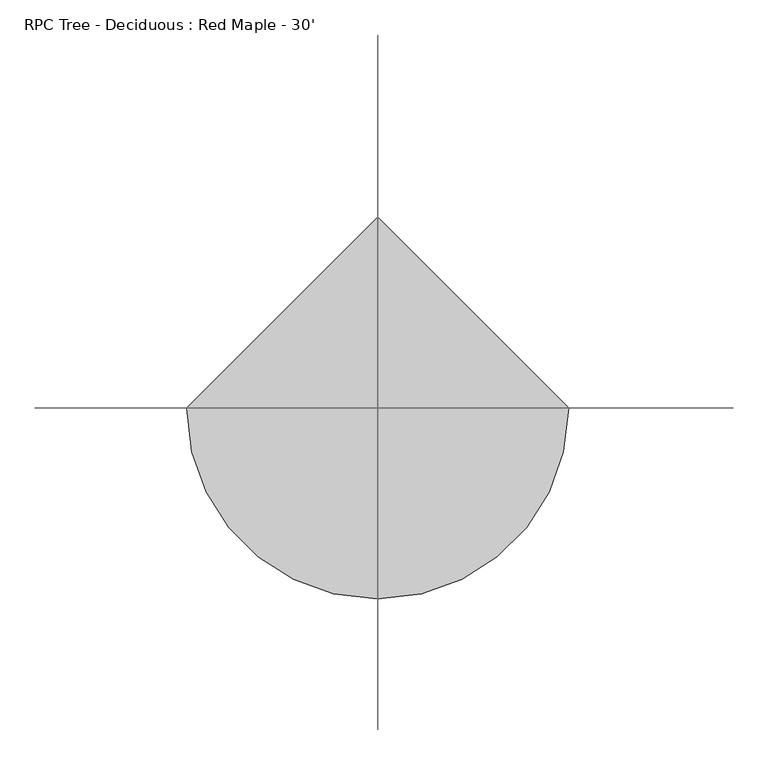
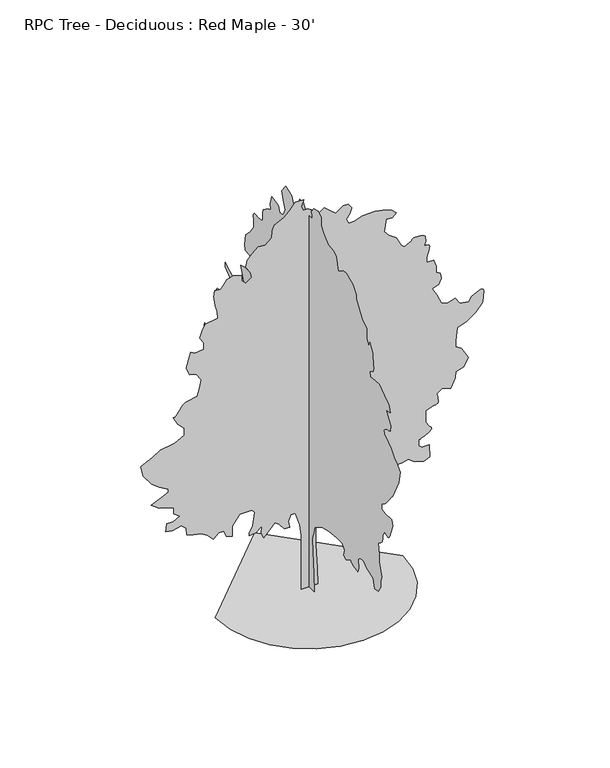
"""IFC4 building model written with IfcOpenShell, lengths in millimetres: geographic element geometry, RPC Tree - Deciduous : Red Maple - 30'."""

import ifcopenshell
import ifcopenshell.guid

model = None  # the IFC model being written
_history = None  # IfcOwnerHistory: only IFC2X3 demands one
_inside = {}  # id of a spatial element -> (the spatial element, [elements in it])
_under = {}  # id of a project, library or spatial element -> (it, [spatial elements below it])
_declared = {}  # id of a project -> (the project, [libraries it declares])
_typed = {}  # id of a type object -> (the type object, [elements of that type])
_made_of = {}  # id of a material, layer set ... -> (it, [elements and type objects made of it])


def new_model(schema):
    """Start an empty IFC model of exactly this schema.

    Asked for "IFC4X3", IfcOpenShell would pick the latest addendum, in which some entities
    have other attributes; the version numbers below select the first issue.
    IFC2X3 requires an IfcOwnerHistory on every rooted entity: one is made here for all.
    """
    global model, _history
    if schema == "IFC4X3":
        model = ifcopenshell.file(schema_version=(4, 3, 0, 0))
    else:
        model = ifcopenshell.file(schema=schema)
    _inside.clear()
    _under.clear()
    _declared.clear()
    _typed.clear()
    _made_of.clear()
    _history = None
    if model.schema == "IFC2X3":
        org = make("IfcOrganization", Name="unknown")
        user = make(
            "IfcPersonAndOrganization",
            ThePerson=make("IfcPerson", FamilyName="unknown"),
            TheOrganization=org,
        )
        app = make(
            "IfcApplication",
            ApplicationDeveloper=org,
            Version="unknown",
            ApplicationFullName="unknown",
            ApplicationIdentifier="unknown",
        )
        _history = make(
            "IfcOwnerHistory",
            OwningUser=user,
            OwningApplication=app,
            ChangeAction="ADDED",
            CreationDate=0,
        )
    return model


def make(cls, **values):
    """One entity of the class cls with the attributes given. An attribute that is None is left unset."""
    return model.create_entity(
        cls, **{name: value for name, value in values.items() if value is not None}
    )


def rooted(cls, **values):
    """An entity with a GlobalId (a new one), such as an element, a storey or a relation."""
    return make(cls, GlobalId=ifcopenshell.guid.new(), OwnerHistory=_history, **values)


def si_unit(unit_type, name, prefix=None):
    """IfcSIUnit, for example si_unit("LENGTHUNIT", "METRE", prefix="MILLI")."""
    return make("IfcSIUnit", UnitType=unit_type, Prefix=prefix, Name=name)


def assignment(units):
    """IfcUnitAssignment: the units of a project."""
    return None if units is None else make("IfcUnitAssignment", Units=units)


def point(xyz):
    """IfcCartesianPoint."""
    return None if xyz is None else make("IfcCartesianPoint", Coordinates=xyz)


def direction(xyz):
    """IfcDirection."""
    return None if xyz is None else make("IfcDirection", DirectionRatios=xyz)


def frame(location, z_axis=None, x_axis=None):
    """IfcAxis2Placement3D, a coordinate frame: its origin and axes. An axis left out is left unset."""
    return make(
        "IfcAxis2Placement3D",
        Location=point(location),
        Axis=direction(z_axis),
        RefDirection=direction(x_axis),
    )


def origin():
    """The frame at (0, 0, 0) with its axes left unset."""
    return frame((0.0, 0.0, 0.0))


def place(relative_to, where):
    """IfcLocalPlacement: puts the frame where relative to a parent placement (None: the world)."""
    return make(
        "IfcLocalPlacement", PlacementRelTo=relative_to, RelativePlacement=where
    )


def context(
    kind, dimensions, precision=None, world=None, true_north=None, identifier=None
):
    """IfcGeometricRepresentationContext, for example the 3D "Model" context."""
    return make(
        "IfcGeometricRepresentationContext",
        ContextIdentifier=identifier,
        ContextType=kind,
        CoordinateSpaceDimension=dimensions,
        Precision=precision,
        WorldCoordinateSystem=world,
        TrueNorth=true_north,
    )


def project(units=None, contexts=None):
    """IfcProject with its units and contexts."""
    return rooted(
        "IfcProject",
        Name="project",
        RepresentationContexts=contexts,
        UnitsInContext=assignment(units),
    )


def spatial(cls, under=None, at=None, **own):
    """A site, building, storey or space (cls), placed at a placement, below another one or the project."""
    s = rooted(cls, ObjectPlacement=at, **own)
    if under is not None:
        _under.setdefault(under.id(), (under, []))[1].append(s)
    return s


def point_list(points):
    """IfcCartesianPointList2D or 3D."""
    cls = (
        "IfcCartesianPointList2D" if len(points[0]) == 2 else "IfcCartesianPointList3D"
    )
    return make(cls, CoordList=points)


def triangles(points, corners, closed=None, point_numbers=None):
    """IfcTriangulatedFaceSet: each triangle names its three corners, points numbered from 1."""
    return make(
        "IfcTriangulatedFaceSet",
        Coordinates=point_list(points),
        Closed=closed,
        CoordIndex=corners,
        PnIndex=point_numbers,
    )


def shape(context_of_items, identifier, shape_type, items):
    """IfcShapeRepresentation: the items that make up one representation, for example the "Body"."""
    return make(
        "IfcShapeRepresentation",
        ContextOfItems=context_of_items,
        RepresentationIdentifier=identifier,
        RepresentationType=shape_type,
        Items=items,
    )


def source(mapping_origin, context_of_items, identifier, shape_type, items):
    """IfcRepresentationMap: a shape defined once, which mapped items show again and again."""
    return make(
        "IfcRepresentationMap",
        MappingOrigin=mapping_origin,
        MappedRepresentation=shape(context_of_items, identifier, shape_type, items),
    )


def transform(
    local_origin,
    x_axis=None,
    y_axis=None,
    z_axis=None,
    scale=None,
    scale2=None,
    scale3=None,
    uniform=True,
):
    """IfcCartesianTransformationOperator3D, or its non-uniform kind. x_axis, y_axis, z_axis: its Axis1, 2, 3."""
    if uniform:
        return make(
            "IfcCartesianTransformationOperator3D",
            Axis1=direction(x_axis),
            Axis2=direction(y_axis),
            LocalOrigin=point(local_origin),
            Scale=scale,
            Axis3=direction(z_axis),
        )
    return make(
        "IfcCartesianTransformationOperator3DnonUniform",
        Axis1=direction(x_axis),
        Axis2=direction(y_axis),
        LocalOrigin=point(local_origin),
        Scale=scale,
        Axis3=direction(z_axis),
        Scale2=scale2,
        Scale3=scale3,
    )


def mapped(mapping_source, mapping_target):
    """IfcMappedItem: shows the shape of a source again, moved by a transform."""
    return make(
        "IfcMappedItem", MappingSource=mapping_source, MappingTarget=mapping_target
    )


def made_of(thing, what):
    """Note that an element or type object is made of a material, layer set ...; save() writes the relation."""
    if what is not None:
        _made_of.setdefault(what.id(), (what, []))[1].append(thing)
    return thing


def element(
    cls,
    number,
    at=None,
    inside=None,
    cuts=None,
    type_object=None,
    material=None,
    context=None,
    identifier="Body",
    shape_type=None,
    held_by="IfcProductDefinitionShape",
    body=None,
    shapes=None,
    **own,
):
    """One element of the class cls, such as IfcWall. Its Tag is "e" and its number.

    at: its placement. inside: the storey or other place that contains it. cuts: it is an
    opening in that element (IfcRelVoidsElement). A single representation is given by context,
    identifier, shape_type and body (its items); several are given by shapes. held_by: the class
    of the entity that holds the representations. save() writes the other relations.
    """
    e = rooted(cls, Tag="e%d" % number, ObjectPlacement=at, **own)
    if body is not None:
        shapes = [shape(context, identifier, shape_type, body)]
    if shapes is not None:
        e.Representation = make(held_by, Representations=shapes)
    if inside is not None:
        _inside.setdefault(inside.id(), (inside, []))[1].append(e)
    if cuts is not None:
        rooted(
            "IfcRelVoidsElement", RelatingBuildingElement=cuts, RelatedOpeningElement=e
        )
    if type_object is not None:
        _typed.setdefault(type_object.id(), (type_object, []))[1].append(e)
    return made_of(e, material)


def aggregate(whole, parts):
    """IfcRelAggregates: a whole, such as a stair, and the parts it consists of."""
    return rooted("IfcRelAggregates", RelatingObject=whole, RelatedObjects=parts)


def save(model, path):
    """Write the relations noted so far, then the file.

    IfcRelAggregates (storeys below a building ...), IfcRelContainedInSpatialStructure (elements
    in a storey), IfcRelDefinesByType, IfcRelAssociatesMaterial and IfcRelDeclares: one each for
    every whole, place, type object, material and project.
    """
    for whole, parts in _under.values():
        aggregate(whole, parts)
    for where, things in _inside.values():
        rooted(
            "IfcRelContainedInSpatialStructure",
            RelatedElements=things,
            RelatingStructure=where,
        )
    for kind, things in _typed.values():
        rooted("IfcRelDefinesByType", RelatedObjects=things, RelatingType=kind)
    for what, things in _made_of.values():
        rooted("IfcRelAssociatesMaterial", RelatedObjects=things, RelatingMaterial=what)
    for by, libraries in _declared.values():
        rooted("IfcRelDeclares", RelatingContext=by, RelatedDefinitions=libraries)
    model.write(path)


def rpc_tree_deciduous_red_maple_30_cba750cc(model_context):
    return source(origin(), model_context, "Body", "Tessellation", [
        triangles([(5.9e-06, 200.5240248, 0.0131599), (5.9e-06, -200.5423013, 0.0131599), (5.9e-06, -173.8047255, 401.079007), (5.9e-06, -147.0663684, 922.4677488), (5.9e-06, -133.6980892, 1216.5822092), (5.9e-06, -173.8047255, 1363.6407475), (5.9e-06, -227.2806583, 1537.4352264), (5.9e-06, -320.8632274, 1590.9124855), (5.9e-06, -534.7644153, 1711.2323215), (5.9e-06, -762.0361897, 1764.7071098), (5.9e-06, -1069.5212002, 1804.8136734), (5.9e-06, -1283.4223881, 1804.8136734), (5.9e-06, -1377.0037399, 1697.8617714), (5.9e-06, -1336.897031, 1550.8033058), (5.9e-06, -1443.848933, 1510.6967422), (5.9e-06, -1617.6460281, 1604.2805649), (5.9e-06, -1620.762553, 1592.8200726), (5.9e-06, -1625.400642, 1581.362051), (5.9e-06, -1633.0790977, 1569.9041748), (5.9e-06, -1645.319339, 1558.4436825), (5.9e-06, -1663.6378429, 1546.9856609), (5.9e-06, -1689.5560284, 1535.5251686), (5.9e-06, -1724.595314, 1524.0672924), (5.9e-06, -1761.1942429, 1514.1662979), (5.9e-06, -1791.4812023, 1507.0721088), (5.9e-06, -1816.5027855, 1502.3197826), (5.9e-06, -1837.3156139, 1499.4343483), (5.9e-06, -1854.971077, 1497.9534794), (5.9e-06, -1870.5234707, 1497.4074371), (5.9e-06, -1885.021859, 1497.3286629), (5.9e-06, -1911.7604885, 1590.9124855), (5.9e-06, -1898.3924091, 1791.445594), (5.9e-06, -1978.6056816, 1871.6588665), (5.9e-06, -2112.293597, 1885.0269459), (5.9e-06, -2219.245499, 1778.0750439), (5.9e-06, -2473.2533958, 1697.8617714), (5.9e-06, -2540.1036758, 1497.3286629), (5.9e-06, -2660.4236572, 1510.6967422), (5.9e-06, -2767.3575371, 1671.125758), (5.9e-06, -2767.3575371, 1804.8136734), (5.9e-06, -2794.1038696, 1911.7655754), (5.9e-06, -2700.5302208, 2219.2479698), (5.9e-06, -2700.5302208, 2393.0450649), (5.9e-06, -2673.7838882, 2660.4236572), (5.9e-06, -2676.8572472, 2660.5759735), (5.9e-06, -2681.2261665, 2661.668058), (5.9e-06, -2688.1603363, 2664.6399696), (5.9e-06, -2698.9553169, 2670.4056061), (5.9e-06, -2714.9066689, 2679.9053169), (5.9e-06, -2737.284082, 2694.1038689), (5.9e-06, -2767.3575371, 2713.8904518), (5.9e-06, -2796.66912, 2738.3761665), (5.9e-06, -2816.8623642, 2765.6558968), (5.9e-06, -2829.4607231, 2795.2721123), (5.9e-06, -2835.9629425, 2826.7681549), (5.9e-06, -2837.9189278, 2859.6612053), (5.9e-06, -2836.8265526, 2893.4940239), (5.9e-06, -2834.2104332, 2927.8096619), (5.9e-06, -2914.423851, 3061.4898743), (5.9e-06, -2945.8434448, 3041.8556076), (5.9e-06, -2976.6790627, 3024.6598549), (5.9e-06, -3006.3211487, 3012.3917084), (5.9e-06, -3034.2357239, 3007.4641022), (5.9e-06, -3059.8135231, 3012.3917084), (5.9e-06, -3082.4449905, 3029.5618813), (5.9e-06, -3101.5964378, 3061.4898743), (5.9e-06, -3235.2766502, 3382.3429642), (5.9e-06, -3195.1700867, 3516.0231766), (5.9e-06, -2941.1698929, 3502.6629456), (5.9e-06, -2794.1038696, 3516.0231766), (5.9e-06, -2807.4641006, 3649.7289688), (5.9e-06, -2841.8811859, 3670.0236603), (5.9e-06, -2876.5523254, 3691.8420959), (5.9e-06, -2911.6551247, 3716.7088921), (5.9e-06, -2947.4692177, 3746.1475021), (5.9e-06, -2984.2230789, 3781.6566719), (5.9e-06, -3022.1707626, 3824.7604362), (5.9e-06, -3061.4898743, 3876.98283), (5.9e-06, -3098.0914192, 3928.4433517), (5.9e-06, -3128.3680595, 3969.3626564), (5.9e-06, -3153.3871719, 4001.5191238), (5.9e-06, -3174.2152611, 4026.6652634), (5.9e-06, -3191.8682533, 4046.5280045), (5.9e-06, -3207.412944, 4062.9110161), (5.9e-06, -3221.9164192, 4077.5159386), (5.9e-06, -3449.1958603, 4532.0748207), (5.9e-06, -3516.0231766, 4826.1815781), (5.9e-06, -3368.9824425, 4986.6084137), (5.9e-06, -3302.1295464, 4999.9686447), (5.9e-06, -3155.0635231, 5187.1415222), (5.9e-06, -3061.4898743, 5253.9944183), (5.9e-06, -3024.5075386, 5271.2916183), (5.9e-06, -2989.023658, 5289.3004028), (5.9e-06, -2956.5878471, 5308.7056137), (5.9e-06, -2928.7238503, 5330.2194168), (5.9e-06, -2906.9559929, 5354.5528152), (5.9e-06, -2892.7574409, 5382.3656525), (5.9e-06, -2887.6775185, 5414.4206726), (5.9e-06, -2894.7134262, 5445.6629517), (5.9e-06, -2914.3474022, 5471.3166183), (5.9e-06, -2944.5228859, 5492.2973145), (5.9e-06, -2983.1054146, 5509.5183563), (5.9e-06, -3028.0125572, 5523.9453827), (5.9e-06, -3077.1107231, 5536.493454), (5.9e-06, -3128.3171906, 5548.100885), (5.9e-06, -3141.7030014, 5695.1669083), (5.9e-06, -3074.850396, 5802.1010788), (5.9e-06, -2967.8906456, 5949.1671021), (5.9e-06, -3128.3171906, 5989.2739563), (5.9e-06, -3074.850396, 6149.7007919), (5.9e-06, -2901.0633293, 6256.6599609), (5.9e-06, -2700.5302208, 6403.7009857), (5.9e-06, -2526.7306549, 6390.3401733), (5.9e-06, -2366.3039646, 6376.9799423), (5.9e-06, -2339.5653351, 6483.9141129), (5.9e-06, -2419.7786076, 6537.4061966), (5.9e-06, -2434.0052101, 6540.4798462), (5.9e-06, -2447.6476913, 6544.8487656), (5.9e-06, -2460.1190231, 6551.7826447), (5.9e-06, -2470.8378456, 6562.577916), (5.9e-06, -2479.217276, 6578.5292679), (5.9e-06, -2484.6730476, 6600.9063904), (5.9e-06, -2486.6238007, 6630.9801361), (5.9e-06, -2485.4529419, 6668.4702896), (5.9e-06, -2482.1813393, 6711.5746353), (5.9e-06, -2477.1522858, 6759.3769501), (5.9e-06, -2470.7209923, 6810.8883408), (5.9e-06, -2463.2380188, 6865.2193268), (5.9e-06, -2455.0515999, 6921.4292679), (5.9e-06, -2446.5172371, 6978.5792679), (5.9e-06, -2339.5653351, 7165.7521454), (5.9e-06, -2299.4587715, 7058.792395), (5.9e-06, -2232.6135784, 7179.1123764), (5.9e-06, -2232.6135784, 7433.1125702), (5.9e-06, -2058.8189541, 7540.0723206), (5.9e-06, -1938.499118, 7700.4985748), (5.9e-06, -1818.1791367, 7874.2856415), (5.9e-06, -1818.1791367, 7967.8845795), (5.9e-06, -1684.4887505, 8128.3114151), (5.9e-06, -1443.848933, 8248.6313965), (5.9e-06, -1310.1610176, 8221.8847733), (5.9e-06, -1136.3639225, 8101.5647919), (5.9e-06, -1042.7825706, 8395.6718399), (5.9e-06, -949.198748, 8462.524736), (5.9e-06, -735.2975601, 8489.2707779), (5.9e-06, -574.8710515, 8649.6976135), (5.9e-06, -467.9217293, 8770.0175949), (5.9e-06, -467.9217293, 8957.1648926), (5.9e-06, -347.6018206, 9037.3780197), (5.9e-06, -187.1730047, 8997.2711655), (5.9e-06, -93.5917073, 8876.9517654), (5.9e-06, -107.5840764, 8845.6589081), (5.9e-06, -119.5886307, 8815.6357407), (5.9e-06, -127.6175737, 8788.2036942), (5.9e-06, -129.6833633, 8764.6324585), (5.9e-06, -123.7979213, 8746.192305), (5.9e-06, -107.9734512, 8734.1779221), (5.9e-06, -80.2224107, 8729.9107407), (5.9e-06, 106.9427183, 8729.9107407), (5.9e-06, 227.262618, 8903.6978073), (5.9e-06, 360.9520595, 8890.3375763), (5.9e-06, 427.7947454, 8729.9107407), (5.9e-06, 601.5918769, 8649.6976135), (5.9e-06, 668.4345629, 8783.3778259), (5.9e-06, 895.7063009, 8876.9517654), (5.9e-06, 1042.7648392, 8676.4180756), (5.9e-06, 975.9195734, 8449.164505), (5.9e-06, 922.4449305, 8302.0984818), (5.9e-06, 989.2901236, 8141.6716461), (5.9e-06, 1122.9781116, 8114.9256042), (5.9e-06, 1176.4527546, 8261.9916275), (5.9e-06, 1443.8312016, 8288.7376694), (5.9e-06, 1497.3083153, 8101.5647919), (5.9e-06, 1470.5696857, 7967.8845795), (5.9e-06, 1590.8896671, 7927.7783066), (5.9e-06, 1764.6841461, 7794.0725143), (5.9e-06, 1778.0546963, 7700.4985748), (5.9e-06, 1778.0546963, 7540.0723206), (5.9e-06, 1844.8974186, 7499.9654663), (5.9e-06, 2005.3239635, 7499.9654663), (5.9e-06, 2036.5838287, 7505.2994431), (5.9e-06, 2066.3221298, 7508.2969345), (5.9e-06, 2093.0200642, 7506.6202927), (5.9e-06, 2115.1586838, 7497.9336136), (5.9e-06, 2131.2167152, 7479.8998306), (5.9e-06, 2139.6749199, 7450.1562973), (5.9e-06, 2139.0144951, 7406.3921082), (5.9e-06, 2134.0639252, 7358.3095779), (5.9e-06, 2130.5182114, 7316.5772415), (5.9e-06, 2128.1407402, 7280.1033051), (5.9e-06, 2126.6979504, 7247.8198105), (5.9e-06, 2125.9562805, 7218.7111221), (5.9e-06, 2125.6844948, 7191.6854462), (5.9e-06, 2125.6464157, 7165.7521454), (5.9e-06, 2259.3343311, 6978.5792679), (5.9e-06, 2433.1289555, 6804.7922012), (5.9e-06, 2473.2356644, 6550.767009), (5.9e-06, 2446.4995056, 6430.4470276), (5.9e-06, 2312.8089741, 6417.0867966), (5.9e-06, 2205.8596882, 6390.3401733), (5.9e-06, 2125.6464157, 6216.5531067), (5.9e-06, 2232.5957016, 6016.0199982), (5.9e-06, 2473.2356644, 6016.0199982), (5.9e-06, 2633.6520355, 5962.5279144), (5.9e-06, 2499.9741486, 5614.9537811), (5.9e-06, 2620.2915138, 5481.2479889), (5.9e-06, 2954.5048347, 5521.3548431), (5.9e-06, 3048.1040634, 5574.8475082), (5.9e-06, 3235.2513611, 5668.4208664), (5.9e-06, 3221.8908394, 5574.8475082), (5.9e-06, 2981.2511673, 5360.9280075), (5.9e-06, 2887.6775185, 5066.8215408), (5.9e-06, 2994.611689, 4839.5420998), (5.9e-06, 3141.6777122, 4852.9279106), (5.9e-06, 3144.9033875, 4867.1011734), (5.9e-06, 3150.3643913, 4880.4869843), (5.9e-06, 3160.2704727, 4892.2217331), (5.9e-06, 3176.8313805, 4901.4926788), (5.9e-06, 3202.2821526, 4907.4870804), (5.9e-06, 3238.8581177, 4909.3921967), (5.9e-06, 3288.7437355, 4906.3947052), (5.9e-06, 3529.3836983, 4879.6486633), (5.9e-06, 3649.703389, 4705.8618874), (5.9e-06, 3609.5968254, 4518.6890099), (5.9e-06, 3462.5308022, 4411.7548393), (5.9e-06, 3342.2108208, 4117.6227928), (5.9e-06, 3395.677906, 3930.4752045), (5.9e-06, 3449.1702805, 3863.622599), (5.9e-06, 3582.8507835, 3636.343158), (5.9e-06, 3850.2367882, 3663.0891998), (5.9e-06, 4024.0235641, 3770.0489502), (5.9e-06, 4077.4906494, 3529.4089874), (5.9e-06, 3823.4904556, 3409.089006), (5.9e-06, 3649.703389, 3355.5966316), (5.9e-06, 3529.3836983, 3088.2362068), (5.9e-06, 3462.5308022, 2927.8096619), (5.9e-06, 3382.3173843, 2700.5302208), (5.9e-06, 3235.2513611, 2727.2762627), (5.9e-06, 3007.9974998, 2767.3831169), (5.9e-06, 2820.8246223, 2727.2762627), (5.9e-06, 2687.1444099, 2513.364901), (5.9e-06, 2860.9311859, 2339.570422), (5.9e-06, 3021.3577309, 2312.8319378), (5.9e-06, 3048.1040634, 2058.8215702), (5.9e-06, 3036.4454727, 2033.2918785), (5.9e-06, 3023.6183487, 2009.2838963), (5.9e-06, 3008.4547394, 1988.3135193), (5.9e-06, 2989.7855301, 1971.9052185), (5.9e-06, 2966.4430595, 1961.5775059), (5.9e-06, 2937.258213, 1958.8496201), (5.9e-06, 2901.0380402, 1965.2402184), (5.9e-06, 2863.2679619, 1977.8690987), (5.9e-06, 2829.7147774, 1992.6010483), (5.9e-06, 2799.6663208, 2009.0882687), (5.9e-06, 2772.4121704, 2026.9800545), (5.9e-06, 2747.2916107, 2045.9209042), (5.9e-06, 2723.5424789, 2065.5651993), (5.9e-06, 2700.504641, 2085.5600544), (5.9e-06, 2606.9309921, 2192.5119564), (5.9e-06, 2589.5829231, 2220.7695339), (5.9e-06, 2571.2947952, 2246.6877193), (5.9e-06, 2551.1527107, 2267.9297367), (5.9e-06, 2528.193647, 2282.1561939), (5.9e-06, 2501.4929512, 2287.0279896), (5.9e-06, 2470.1189941, 2280.208057), (5.9e-06, 2433.1289555, 2259.3571495), (5.9e-06, 2386.7865807, 2232.2681053), (5.9e-06, 2329.2174202, 2207.9857212), (5.9e-06, 2262.2959236, 2186.0425838), (5.9e-06, 2187.8891281, 2165.9689545), (5.9e-06, 2107.8714832, 2147.2998905), (5.9e-06, 2024.1123516, 2129.5656532), (5.9e-06, 1938.4812412, 2112.2986839), (5.9e-06, 1724.5775826, 2058.8215702), (5.9e-06, 1791.4227757, 1925.1335094), (5.9e-06, 2005.3239635, 1791.445594), (5.9e-06, 2112.2758656, 1617.6484989), (5.9e-06, 1925.1106911, 1550.8033058), (5.9e-06, 1899.2305847, 1550.9989334), (5.9e-06, 1872.766357, 1552.362949), (5.9e-06, 1845.1311253, 1556.0662113), (5.9e-06, 1815.7433842, 1563.2772537), (5.9e-06, 1784.0161057, 1575.1644642), (5.9e-06, 1749.3654591, 1592.8988468), (5.9e-06, 1711.2095032, 1617.6484989), (5.9e-06, 1671.8826885, 1646.6858253), (5.9e-06, 1633.9579685, 1676.4242718), (5.9e-06, 1597.2041073, 1706.7493103), (5.9e-06, 1561.3849274, 1737.539146), (5.9e-06, 1526.2668674, 1768.6821579), (5.9e-06, 1491.6162209, 1800.0587311), (5.9e-06, 1457.1991356, 1831.5523029), (5.9e-06, 1189.8233047, 1911.7655754), (5.9e-06, 975.9195734, 1951.872139), (5.9e-06, 762.0183855, 2005.3467819), (5.9e-06, 548.1146542, 1965.2402184), (5.9e-06, 253.9999576, 1858.2883163), (5.9e-06, 173.7866851, 1751.3390305), (5.9e-06, 106.9427183, 1564.173856), (5.9e-06, 80.2041161, 1296.7955544), (5.9e-06, 106.9427183, 935.8358282), (5.9e-06, 160.4173885, 414.4495934), (-2085.2019367, 0.0, 0.0), (-2030.0762318, -477.7896226, 0.0), (-1873.078838, -916.5648388, 0.0), (-1626.7799183, -1303.7500717, 0.0), (-1303.7500717, -1626.7799183, 0.0), (-916.5648388, -1873.078838, 0.0), (-477.7896226, -2030.0762318, 0.0), (9.11e-05, -2085.2019367, 0.0), (477.7896226, -2030.0762318, 0.0), (916.5648388, -1873.078838, 0.0), (1303.7500717, -1626.7799183, 0.0), (1626.7799183, -1303.7500717, 0.0), (1873.078838, -916.5648388, 0.0), (2030.0762318, -477.7896226, 0.0), (2085.2019367, 0.0001828, 0.0), (-0.0002734, 2085.2019367, 0.0), (199.8874902, 0.0002285, 0.005264), (-169.704903, 0.0002285, 0.005264), (-169.704903, 0.0001919, 684.4365658), (-169.704903, 0.0001645, 1040.3416586), (-169.704903, 0.0001554, 1273.0464226), (-210.770892, 0.0001371, 1533.1325821), (-306.5909517, 0.0001188, 1834.2801888), (-402.4125375, 0.0001188, 1834.2801888), (-457.1673348, 0.0001279, 1683.7063854), (-429.7886644, 0.0001371, 1546.8205547), (-552.9863771, 0.0001371, 1560.5086727), (-662.4960445, 0.0001279, 1697.3945034), (-758.317594, 0.0001279, 1765.8374187), (-867.8247179, 0.0001279, 1642.639706), (-1004.7104759, 0.0001371, 1505.7538754), (-1059.465346, 0.0001371, 1628.9515881), (-1045.777228, 0.0001279, 1793.2159801), (-1182.6630587, 0.0001279, 1683.7063854), (-1333.2394054, 0.0001279, 1670.0182674), (-1333.2394054, 0.0001279, 1738.4611828), (-1251.1059013, 0.0001188, 1875.3470135), (-1210.0416927, 0.0001005, 2176.4972363), (-1278.4846081, 0.0001005, 2244.9401516), (-1538.5681515, 0.0001005, 2244.9401516), (-1702.8300728, 0.0001097, 2012.2328442), (-1702.8300728, 0.0001188, 1916.4136929), (-1702.8300728, 0.0001279, 1779.5280075), (-1839.7183743, 0.0001188, 1834.2801888), (-1894.4731716, 0.0001097, 1971.1686356), (-2003.9802956, 0.0001097, 1971.1686356), (-2127.1780083, 0.0001188, 1861.6588955), (-2264.063839, 0.0001097, 1998.5447262), (-2400.9521404, 0.0001097, 2080.6756142), (-2578.9149696, 0.0001005, 2121.7424389), (-2715.7955681, 0.0001005, 2176.4972363), (-2729.4863022, 9.14e-05, 2327.0711849), (-2838.9857231, 8.22e-05, 2422.8926617), (-3044.3194107, 9.14e-05, 2381.8259823), (-3181.2000092, 8.22e-05, 2409.204689), (-3167.5095657, 7.31e-05, 2587.1444092), (-3016.9382332, 7.31e-05, 2587.1444092), (-2880.0576347, 7.31e-05, 2669.2882324), (-3003.2474991, 6.4e-05, 2765.0969193), (-3003.2474991, 5.48e-05, 2902.0030975), (-3140.1283882, 5.48e-05, 2956.7401634), (-3331.7713417, 5.48e-05, 3011.5025185), (-3509.7241425, 4.57e-05, 3148.3834076), (-3290.6997208, 3.66e-05, 3244.2176743), (-3126.4376541, 3.66e-05, 3312.6451836), (-3126.4376541, 2.74e-05, 3381.0982727), (-3331.7713417, 1.83e-05, 3504.2884277), (-3496.0334084, 1.83e-05, 3627.5038719), (-3687.6766525, 0.0, 3887.5746254), (-3742.4390076, -1.83e-05, 4133.9802246), (-3632.9395866, -1.83e-05, 4188.7172905), (-3482.3426743, -2.74e-05, 4257.1703796), (-3304.3901642, -2.74e-05, 4366.6698006), (-2989.5570557, -3.66e-05, 4421.4324463), (-2770.532634, -3.66e-05, 4530.9318672), (-2770.532634, -4.57e-05, 4695.1936432), (-2921.1292557, -5.48e-05, 4845.7905556), (-3016.9382332, -7.31e-05, 5023.742775), (-3007.9974998, -7.31e-05, 5021.1266556), (-2998.2184456, -7.31e-05, 5020.5679688), (-2986.7630402, -7.31e-05, 5024.0985672), (-2972.7929626, -7.31e-05, 5033.6997253), (-2955.4701828, -7.31e-05, 5051.4544556), (-2933.9816689, -7.31e-05, 5079.3946106), (-2907.4388123, -7.31e-05, 5119.5520432), (-2879.295472, -7.31e-05, 5162.0971207), (-2853.3113022, -8.22e-05, 5196.7426804), (-2829.1305107, -8.22e-05, 5224.783992), (-2806.3720161, -8.22e-05, 5247.5680664), (-2784.7058968, -8.22e-05, 5266.4145905), (-2763.7507805, -8.22e-05, 5282.6199966), (-2743.1767456, -8.22e-05, 5297.5045532), (-2483.0830284, -9.14e-05, 5352.2669083), (-2428.328231, -0.0001005, 5543.9098618), (-2400.9521404, -0.0001097, 5708.1719284), (-2510.4618805, -0.0001188, 5872.4339951), (-2647.3424789, -0.0001188, 5913.4803268), (-2729.4863022, -0.0001371, 6091.4328369), (-2674.7236565, -0.0001462, 6283.0757904), (-2633.6520355, -0.0001554, 6433.6474136), (-2537.8378258, -0.0001462, 6378.9100571), (-2346.1973431, -0.0001554, 6406.2915253), (-2346.1973431, -0.0001645, 6556.8625671), (-2428.328231, -0.0001645, 6693.7437469), (-2373.5734337, -0.0001736, 6844.3147888), (-2305.1305183, -0.0001828, 6981.1953873), (-2031.3590023, -0.0001919, 7022.2672989), (-2045.0471203, -0.0002011, 7186.5293655), (-2086.1137997, -0.0002102, 7337.1004074), (-2113.4900356, -0.0002193, 7556.1248291), (-2099.8019176, -0.0002285, 7693.0060089), (-1962.916087, -0.0002285, 7679.3149841), (-1894.4731716, -0.0002285, 7761.4588074), (-1826.0302563, -0.0002376, 7857.2674942), (-1689.1419548, -0.0002376, 7898.3394058), (-1497.5013268, -0.0002376, 7843.5770508), (-1497.5013268, -0.0002285, 7720.3868958), (-1401.6823208, -0.0002285, 7624.5782089), (-1278.4846081, -0.0002285, 7720.3868958), (-1305.8606987, -0.0002376, 7857.2674942), (-1401.6823208, -0.0002467, 8007.8391174), (-1374.303614, -0.0002559, 8158.4357391), (-1264.7940193, -0.000265, 8267.9354507), (-1127.9081886, -0.0002742, 8391.1250244), (-977.3343853, -0.000265, 8377.434581), (-826.7605093, -0.0002742, 8500.6503159), (-813.0699205, -0.0002833, 8651.2213577), (-772.0057119, -0.0002924, 8774.4115128), (-566.6744588, -0.0003016, 8870.2457794), (-443.4767461, -0.0003016, 8979.745491), (-306.5909517, -0.0003107, 9144.0075577), (-114.9505871, -0.0003107, 9144.0075577), (-169.704903, -0.0003016, 8993.4359344), (-128.6391684, -0.0003016, 8897.6016678), (-32.8188589, -0.0003016, 8897.6016678), (49.3128694, -0.0002924, 8842.8648926), (76.6900319, -0.0002924, 8733.3396011), (240.9532249, -0.0002924, 8719.6491577), (336.7737751, -0.0002924, 8788.1019562), (473.6595695, -0.0002833, 8678.6028259), (596.8572822, -0.0002833, 8569.0781158), (761.1217833, -0.0002833, 8692.2932693), (870.6314507, -0.0002833, 8692.2932693), (952.7624113, -0.0002833, 8582.7685593), (911.6956593, -0.0002742, 8445.8879608), (829.5646986, -0.000265, 8350.0786926), (884.319496, -0.000265, 8240.5539825), (1007.5172087, -0.000265, 8240.5539825), (1199.1578367, -0.000265, 8309.006781), (1472.9294254, -0.000265, 8309.006781), (1637.1938175, -0.000265, 8281.6258942), (1842.5225636, -0.0002559, 8213.1725143), (1938.3441856, -0.0002559, 8117.3638275), (1856.2106815, -0.0002467, 8021.5295609), (1719.3248508, -0.0002467, 8035.2200043), (1691.9487602, -0.0002376, 7912.0298492), (1678.2580261, -0.0002285, 7761.4588074), (1774.0796482, -0.0002285, 7638.2686523), (1938.3441856, -0.0002193, 7528.7439423), (2047.8513096, -0.0002011, 7309.7195206), (2116.2940796, -0.0002011, 7254.982164), (2280.558617, -0.0002102, 7337.1004074), (2283.7919952, -0.0002102, 7348.7589981), (2288.8187233, -0.0002102, 7359.9350601), (2297.439418, -0.0002102, 7370.1460648), (2311.4475746, -0.0002102, 7378.9344818), (2332.6388683, -0.0002102, 7385.7927841), (2362.8089745, -0.0002102, 7390.2628601), (2403.7563297, -0.0002102, 7391.8633438), (2446.2989365, -0.0002102, 7390.2628601), (2480.9392639, -0.0002102, 7385.7927841), (2508.9962723, -0.0002102, 7378.9344818), (2531.7826721, -0.0002102, 7370.1460648), (2550.619313, -0.0002102, 7359.9350601), (2566.8244286, -0.0002102, 7348.7589981), (2581.7089851, -0.0002102, 7337.1004074), (2595.3994286, -0.0002011, 7213.9108337), (2568.018251, -0.0001919, 7118.1015656), (2599.8953751, -0.0001919, 7117.6446167), (2629.5115906, -0.0001919, 7114.5709671), (2654.581572, -0.0001919, 7106.2400803), (2672.8188309, -0.0001919, 7089.9840958), (2681.9627495, -0.0001919, 7063.2124741), (2679.7274208, -0.0001919, 7023.2579361), (2663.8525177, -0.0001828, 6967.5049438), (2643.9641968, -0.0001828, 6908.5771454), (2630.5530968, -0.0001828, 6859.6818741), (2622.5268425, -0.0001736, 6819.1686493), (2618.8183479, -0.0001736, 6785.3614105), (2618.3358192, -0.0001736, 6756.6085144), (2620.0121704, -0.0001736, 6731.1833221), (2622.7806061, -0.0001736, 6707.4341904), (2773.3519386, -0.0001736, 6707.4341904), (2828.1145844, -0.0001554, 6543.1721237), (2828.1145844, -0.0001554, 6406.2915253), (2923.9232712, -0.0001462, 6351.5291702), (2937.6140053, -0.0001371, 6228.3390152), (2882.8516502, -0.0001371, 6105.1232803), (2745.9707611, -0.0001279, 6050.3865051), (2841.8050278, -0.0001188, 5872.4339951), (2937.6140053, -0.0001097, 5653.4095734), (3074.4946037, -0.0001005, 5584.9561935), (3252.4471138, -0.0001097, 5639.7191299), (3348.2813805, -0.0001005, 5489.1475067), (3553.5897789, -9.14e-05, 5461.7666199), (3622.042868, -0.0001005, 5557.5753067), (3677.3894897, -0.0001005, 5589.3251129), (3730.4754936, -0.0001005, 5617.7989563), (3779.0149727, -0.0001097, 5639.8458664), (3820.6964401, -0.0001097, 5652.1648819), (3853.3101471, -0.0001097, 5651.5806152), (3874.5446068, -0.0001097, 5634.8165222), (3882.1392014, -0.0001005, 5598.6472183), (3881.3261696, -0.0001005, 5553.3081253), (3879.0911316, -0.0001005, 5510.8647858), (3875.6619804, -9.14e-05, 5470.7835114), (3871.2677719, -9.14e-05, 5432.6323517), (3866.1625603, -9.14e-05, 5395.9293594), (3860.5745293, -9.14e-05, 5360.1664261), (3854.7580238, -9.14e-05, 5324.8854401), (3704.1866913, -7.31e-05, 5160.6239548), (3512.5434471, -6.4e-05, 5010.0523315), (3293.5190254, -6.4e-05, 4941.5995331), (3266.1378479, -4.57e-05, 4640.4565773), (3266.1378479, -3.66e-05, 4503.5506897), (3389.3280029, -3.66e-05, 4421.4324463), (3539.9246246, -1.83e-05, 4161.336113), (3444.090358, -9.1e-06, 3969.7184486), (3266.1378479, 0.0, 3914.9558029), (3252.4471138, 9.1e-06, 3778.0752045), (3156.638427, 1.83e-05, 3559.0507828), (2964.9951828, 1.83e-05, 3627.5038719), (2846.3771324, 1.83e-05, 3536.8765549), (2845.4879425, 1.83e-05, 3538.3244316), (2845.1071518, 1.83e-05, 3537.5369797), (2845.7675766, 1.83e-05, 3532.3047409), (2847.9773254, 1.83e-05, 3520.3665161), (2852.269796, 1.83e-05, 3499.5131378), (2859.1786766, 2.74e-05, 3467.5345665), (2869.1609161, 2.74e-05, 3422.1701843), (2875.307634, 2.74e-05, 3376.1453773), (2871.3959541, 2.74e-05, 3342.3378479), (2859.1025185, 3.66e-05, 3318.7157433), (2840.1286766, 3.66e-05, 3303.2219215), (2816.1002014, 3.66e-05, 3293.8492378), (2788.7190239, 3.66e-05, 3288.5405502), (2759.6614952, 3.66e-05, 3285.264006), (2595.3994286, 3.66e-05, 3230.5269402), (2595.3994286, 5.48e-05, 2956.7401634), (2677.517672, 6.4e-05, 2833.5500084), (2697.53302, 6.4e-05, 2815.871727), (2714.297113, 6.4e-05, 2797.7106262), (2724.5839851, 6.4e-05, 2778.5844681), (2725.1682518, 6.4e-05, 2758.0357224), (2712.8492363, 6.4e-05, 2735.582151), (2684.3503944, 7.31e-05, 2710.7156456), (2636.4713402, 7.31e-05, 2682.9786758), (2584.1727882, 7.31e-05, 2657.2229805), (2543.4055092, 7.31e-05, 2637.9697952), (2512.1864845, 7.31e-05, 2624.0761665), (2488.640538, 7.31e-05, 2614.5002975), (2470.8427872, 7.31e-05, 2608.1503944), (2456.8753258, 7.31e-05, 2603.9593712), (2444.8231544, 7.31e-05, 2600.8351433), (2444.8231544, 8.22e-05, 2463.9594864), (2513.2660698, 9.14e-05, 2395.5139549), (2677.517672, 9.14e-05, 2395.5139549), (2691.2084061, 0.0001005, 2108.0543209), (2554.3275169, 0.0001097, 2053.2995235), (2349.0015324, 0.0001005, 2121.7424389), (2212.1157017, 0.0001005, 2217.564061), (2075.229871, 0.0001005, 2190.1853542), (1828.8344456, 0.0001005, 2176.4972363), (1678.2580261, 0.0001005, 2135.4305569), (1664.5700535, 0.0001188, 1943.7899288), (1513.9961048, 0.0001188, 1930.1018108), (1322.3554768, 0.0001188, 1943.7899288), (1240.2219727, 0.0001188, 1820.5922161), (952.7624113, 0.0001279, 1779.5280075), (733.7430765, 0.0001188, 1834.2801888), (733.7430765, 0.0001371, 1615.2634701), (555.7930736, 0.0001371, 1628.9515881), (501.0382762, 0.0001279, 1738.4611828), (405.2166904, 0.0001279, 1697.3945034), (295.7070412, 0.0001279, 1697.3945034), (254.6428326, 0.0001188, 1820.5922161), (145.13292, 0.0001279, 1697.3945034), (131.4443387, 0.0001371, 1546.8205547), (145.13292, 0.0001554, 1314.1132473), (145.13292, 0.0001736, 930.8319912), (186.1989181, 0.0002102, 383.2863067)], [[130, 131, 132], [208, 209, 210], [208, 210, 211], [207, 208, 211], [230, 231, 232], [230, 232, 233], [276, 277, 278], [229, 230, 233], [229, 233, 234], [302, 1, 2], [302, 2, 3], [302, 3, 4], [301, 302, 4], [301, 4, 5], [300, 301, 5], [300, 5, 6], [299, 300, 6], [299, 6, 7], [108, 109, 110], [203, 204, 205], [206, 207, 211], [206, 211, 212], [108, 110, 111], [202, 203, 205], [13, 14, 15], [13, 15, 16], [236, 237, 238], [171, 172, 173], [170, 171, 173], [170, 173, 174], [36, 37, 38], [36, 38, 39], [36, 39, 40], [275, 276, 278], [275, 278, 279], [275, 279, 280], [275, 280, 281], [275, 281, 282], [275, 282, 283], [275, 283, 284], [275, 284, 285], [275, 285, 286], [275, 286, 287], [275, 287, 288], [275, 288, 289], [275, 289, 290], [274, 275, 290], [274, 290, 291], [274, 291, 292], [67, 68, 69], [66, 67, 69], [164, 165, 166], [164, 166, 167], [163, 164, 167], [163, 167, 168], [242, 243, 244], [29, 30, 31], [104, 105, 106], [197, 198, 199], [28, 29, 31], [298, 299, 7], [66, 69, 70], [65, 66, 70], [64, 65, 70], [63, 64, 70], [62, 63, 70], [61, 62, 70], [60, 61, 70], [59, 60, 70], [27, 28, 31], [150, 151, 152], [160, 161, 162], [159, 160, 162], [196, 197, 199], [195, 196, 199], [195, 199, 200], [26, 27, 31], [133, 134, 135], [242, 244, 245], [242, 245, 246], [242, 246, 247], [242, 247, 248], [242, 248, 249], [242, 249, 250], [242, 250, 251], [242, 251, 252], [242, 252, 253], [242, 253, 254], [242, 254, 255], [242, 255, 256], [242, 256, 257], [242, 257, 258], [242, 258, 259], [241, 242, 259], [241, 259, 260], [241, 260, 261], [241, 261, 262], [241, 262, 263], [241, 263, 264], [298, 7, 8], [274, 292, 293], [147, 148, 149], [147, 149, 150], [147, 150, 152], [147, 152, 153], [147, 153, 154], [147, 154, 155], [147, 155, 156], [36, 40, 41], [36, 41, 42], [35, 36, 42], [34, 35, 42], [34, 42, 43], [86, 87, 88], [86, 88, 89], [34, 43, 44], [104, 106, 107], [103, 104, 107], [102, 103, 107], [25, 26, 31], [25, 31, 32], [24, 25, 32], [23, 24, 32], [22, 23, 32], [21, 22, 32], [20, 21, 32], [19, 20, 32], [18, 19, 32], [17, 18, 32], [16, 17, 32], [13, 16, 32], [12, 13, 32], [102, 107, 108], [101, 102, 108], [129, 130, 132], [146, 147, 156], [100, 101, 108], [236, 238, 239], [146, 156, 157], [221, 222, 223], [221, 223, 224], [221, 224, 225], [220, 221, 225], [219, 220, 225], [218, 219, 225], [217, 218, 225], [216, 217, 225], [215, 216, 225], [214, 215, 225], [213, 214, 225], [213, 225, 226], [33, 34, 44], [235, 236, 239], [298, 8, 9], [297, 298, 9], [12, 32, 33], [58, 59, 70], [175, 176, 177], [85, 86, 89], [85, 89, 90], [85, 90, 91], [85, 91, 92], [84, 85, 92], [84, 92, 93], [83, 84, 93], [82, 83, 93], [82, 93, 94], [81, 82, 94], [80, 81, 94], [80, 94, 95], [79, 80, 95], [12, 33, 44], [78, 79, 95], [77, 78, 95], [76, 77, 95], [75, 76, 95], [74, 75, 95], [73, 74, 95], [72, 73, 95], [71, 72, 95], [71, 95, 96], [108, 111, 112], [108, 112, 113], [100, 108, 113], [100, 113, 114], [99, 100, 114], [98, 99, 114], [194, 195, 200], [128, 129, 132], [137, 138, 139], [175, 177, 178], [174, 175, 178], [241, 264, 265], [139, 140, 141], [139, 141, 142], [137, 139, 142], [229, 234, 235], [229, 235, 239], [228, 229, 239], [227, 228, 239], [227, 239, 240], [226, 227, 240], [213, 226, 240], [136, 137, 142], [142, 143, 144], [142, 144, 145], [145, 146, 157], [127, 128, 132], [11, 12, 44], [170, 174, 178], [194, 200, 201], [71, 96, 97], [145, 157, 158], [169, 170, 178], [212, 213, 240], [206, 212, 240], [205, 206, 240], [205, 240, 241], [205, 241, 265], [205, 265, 266], [205, 266, 267], [205, 267, 268], [205, 268, 269], [205, 269, 270], [205, 270, 271], [205, 271, 272], [205, 272, 273], [205, 273, 274], [205, 274, 293], [205, 293, 294], [205, 294, 295], [202, 205, 295], [202, 295, 296], [201, 202, 296], [201, 296, 297], [201, 297, 9], [201, 9, 10], [201, 10, 11], [201, 11, 44], [194, 201, 44], [193, 194, 44], [193, 44, 45], [193, 45, 46], [193, 46, 47], [193, 47, 48], [193, 48, 49], [193, 49, 50], [193, 50, 51], [193, 51, 52], [193, 52, 53], [193, 53, 54], [193, 54, 55], [193, 55, 56], [193, 56, 57], [193, 57, 58], [193, 58, 70], [193, 70, 71], [193, 71, 97], [193, 97, 98], [193, 98, 114], [193, 114, 115], [192, 193, 115], [191, 192, 115], [190, 191, 115], [189, 190, 115], [188, 189, 115], [187, 188, 115], [186, 187, 115], [185, 186, 115], [184, 185, 115], [183, 184, 115], [182, 183, 115], [181, 182, 115], [180, 181, 115], [179, 180, 115], [178, 179, 115], [169, 178, 115], [168, 169, 115], [163, 168, 115], [162, 163, 115], [159, 162, 115], [158, 159, 115], [145, 158, 115], [142, 145, 115], [136, 142, 115], [135, 136, 115], [133, 135, 115], [132, 133, 115], [127, 132, 115], [126, 127, 115], [126, 115, 116], [125, 126, 116], [124, 125, 116], [123, 124, 116], [122, 123, 116], [121, 122, 116], [121, 116, 117], [120, 121, 117], [120, 117, 118], [119, 120, 118], [317, 318, 303], [316, 317, 303], [316, 303, 304], [315, 316, 304], [315, 304, 305], [315, 305, 306], [314, 315, 306], [313, 314, 306], [313, 306, 307], [313, 307, 308], [313, 308, 309], [313, 309, 310], [313, 310, 311], [313, 311, 312], [379, 380, 381], [379, 381, 382], [364, 365, 366], [344, 345, 346], [332, 333, 334], [433, 434, 435], [327, 328, 329], [401, 402, 403], [327, 329, 330], [344, 346, 347], [343, 344, 347], [332, 334, 335], [432, 433, 435], [379, 382, 383], [534, 535, 536], [336, 337, 338], [336, 338, 339], [335, 336, 339], [582, 583, 584], [582, 584, 585], [593, 319, 320], [593, 320, 321], [592, 593, 321], [592, 321, 322], [591, 592, 322], [591, 322, 323], [412, 413, 414], [331, 332, 335], [591, 323, 324], [590, 591, 324], [568, 569, 570], [568, 570, 571], [568, 571, 572], [568, 572, 573], [567, 568, 573], [348, 349, 350], [532, 533, 534], [454, 455, 456], [454, 456, 457], [453, 454, 457], [357, 358, 359], [356, 357, 359], [355, 356, 359], [355, 359, 360], [363, 364, 366], [363, 366, 367], [589, 590, 324], [589, 324, 325], [576, 577, 578], [371, 372, 373], [335, 339, 340], [379, 383, 384], [504, 505, 506], [440, 441, 442], [417, 418, 419], [326, 327, 330], [494, 495, 496], [586, 587, 588], [362, 363, 367], [432, 435, 436], [588, 589, 325], [326, 330, 331], [352, 353, 354], [585, 586, 588], [452, 453, 457], [331, 335, 340], [379, 384, 385], [416, 417, 419], [415, 416, 419], [411, 412, 414], [531, 532, 534], [528, 529, 530], [528, 530, 531], [527, 528, 531], [431, 432, 436], [414, 415, 419], [411, 414, 419], [411, 419, 420], [410, 411, 420], [409, 410, 420], [576, 578, 579], [371, 373, 374], [370, 371, 374], [370, 374, 375], [369, 370, 375], [369, 375, 376], [368, 369, 376], [368, 376, 377], [407, 408, 409], [452, 457, 458], [451, 452, 458], [450, 451, 458], [450, 458, 459], [497, 498, 499], [497, 499, 500], [497, 500, 501], [445, 446, 447], [444, 445, 447], [443, 444, 447], [443, 447, 448], [326, 331, 340], [360, 361, 362], [494, 496, 497], [405, 406, 407], [405, 407, 409], [398, 399, 400], [398, 400, 401], [398, 401, 403], [398, 403, 404], [397, 398, 404], [579, 580, 581], [494, 497, 501], [425, 426, 427], [379, 385, 386], [429, 430, 431], [527, 531, 534], [477, 478, 479], [476, 477, 479], [475, 476, 479], [474, 475, 479], [473, 474, 479], [473, 479, 480], [472, 473, 480], [471, 472, 480], [470, 471, 480], [469, 470, 480], [468, 469, 480], [467, 468, 480], [466, 467, 480], [465, 466, 480], [464, 465, 480], [463, 464, 480], [566, 567, 573], [566, 573, 574], [566, 574, 575], [428, 429, 431], [428, 431, 436], [422, 423, 424], [422, 424, 425], [422, 425, 427], [421, 422, 427], [342, 343, 347], [437, 438, 439], [436, 437, 439], [428, 436, 439], [378, 379, 386], [378, 386, 387], [378, 387, 388], [378, 388, 389], [378, 389, 390], [378, 390, 391], [378, 391, 392], [378, 392, 393], [378, 393, 394], [378, 394, 395], [582, 585, 588], [351, 352, 354], [513, 514, 515], [512, 513, 515], [511, 512, 515], [511, 515, 516], [510, 511, 516], [510, 516, 517], [509, 510, 517], [509, 517, 518], [509, 518, 519], [508, 509, 519], [507, 508, 519], [507, 519, 520], [507, 520, 521], [507, 521, 522], [507, 522, 523], [507, 523, 524], [506, 507, 524], [506, 524, 525], [504, 506, 525], [503, 504, 525], [354, 355, 360], [579, 581, 582], [342, 347, 348], [342, 348, 350], [342, 350, 351], [342, 351, 354], [342, 354, 360], [342, 360, 362], [342, 362, 367], [342, 367, 368], [342, 368, 377], [341, 342, 377], [449, 450, 459], [527, 534, 536], [404, 405, 409], [341, 377, 378], [341, 378, 395], [341, 395, 396], [503, 525, 526], [440, 442, 443], [555, 556, 557], [554, 555, 557], [554, 557, 558], [553, 554, 558], [552, 553, 558], [552, 558, 559], [551, 552, 559], [551, 559, 560], [551, 560, 561], [551, 561, 562], [551, 562, 563], [551, 563, 564], [551, 564, 565], [551, 565, 566], [551, 566, 575], [550, 551, 575], [550, 575, 576], [460, 461, 462], [483, 484, 485], [482, 483, 485], [482, 485, 486], [481, 482, 486], [481, 486, 487], [480, 481, 487], [480, 487, 488], [463, 480, 488], [463, 488, 489], [463, 489, 490], [463, 490, 491], [463, 491, 492], [463, 492, 493], [463, 493, 494], [463, 494, 501], [341, 396, 397], [340, 341, 397], [326, 340, 397], [325, 326, 397], [588, 325, 397], [582, 588, 397], [579, 582, 397], [576, 579, 397], [550, 576, 397], [550, 397, 404], [550, 404, 409], [550, 409, 420], [550, 420, 421], [549, 550, 421], [549, 421, 427], [549, 427, 428], [549, 428, 439], [549, 439, 440], [549, 440, 443], [549, 443, 448], [549, 448, 449], [549, 449, 459], [549, 459, 460], [549, 460, 462], [549, 462, 463], [549, 463, 501], [549, 501, 502], [549, 502, 503], [548, 549, 503], [547, 548, 503], [526, 527, 536], [503, 526, 536], [544, 545, 546], [543, 544, 546], [543, 546, 547], [542, 543, 547], [541, 542, 547], [540, 541, 547], [503, 536, 537], [547, 503, 537], [547, 537, 538], [547, 538, 539], [540, 547, 539]], closed=False),
    ])


if __name__ == "__main__":
    model = new_model("IFC4")
    model_context = context("Model", 3, world=origin())
    ifc_project = project(units=[si_unit("LENGTHUNIT", "METRE", prefix="MILLI")], contexts=[model_context])
    site = spatial("IfcSite", under=ifc_project)
    building = spatial("IfcBuilding", under=site)
    placement = place(None, origin())
    rpc_tree_deciduous_red_maple_30_shape = rpc_tree_deciduous_red_maple_30_cba750cc(model_context)
    element("IfcGeographicElement", 1, ObjectType="RPC Tree - Deciduous : Red Maple - 30'", at=placement, inside=building, context=model_context, shape_type="MappedRepresentation", body=[
        mapped(rpc_tree_deciduous_red_maple_30_shape, transform((0.0, 0.0, 0.0), x_axis=(1.0, 0.0, 0.0), y_axis=(0.0, 1.0, 0.0), z_axis=(0.0, 0.0, 1.0))),
    ])
    save(model, "model.ifc")

# Revit data of these elements
# Type "RPC Tree - Deciduous : Red Maple - 30'"
#   built-in parameter 1005198 = "{2, 15},{39, RPC-16-G0SR-83PX-Q347-6000-ST1L-LVER-AU},{1, 0},{1, 0},{2, 13},{1, 8},{5, Color},{1, 0},{1, 0},{3, 0.8},{3, 0.8},{3, 0.8},{1, 8},{7, BBoxMin},{1, 0},{1, 0},{1, 0},{1, 0},{1, 0},{1, 8},{7, BBoxMax},{1, 0},{1, 0},{1, 0},{1, 0},{1, 0},{2, 11},{9, RPCTypeId},{1, 0},{1, 0},{39, RPC-16-G0SR-83PX-Q347-6000-ST1L-LVER-AU},{1, 6},{14, RPCPlantHeight},{1, 0},{1, 0},{2, 30},{2, 11},{7, keyword},{1, 0},{1, 0},{34, :RPCs:Trees [General]:Geometry:RPC},{2, 11},{8, category},{1, 0},{1, 0},{15, Trees [General]},{2, 11},{12, LocalizedUID},{1, 0},{1, 0},{9, Red Maple},{2, 14},{6, Height},{1, 0},{1, 0},{2, 30},{1, 2},{16, Cast Reflections},{1, 0},{1, 0},{1, 0},{1, 2},{12, Cast Shadows},{1, 0},{1, 0},{1, 1},{1, 2},{9, Lock View},{1, 0},{1, 0},{1, 0},{1, 4},{5, ViewC},{1, 0},{1, 0},{1, 0},{21, assetlibrary_base.fbx},{1, 5},"
#   built-in parameter 1005195 = "RPC-16-G0SR-83PX-Q347-6000-ST1L-LVER-AU"
#   Type Comments = "Red Maple"
#   Assembly Code = "G2050500"
#   Height = 30' - 0"
#   Default Elevation = 0
